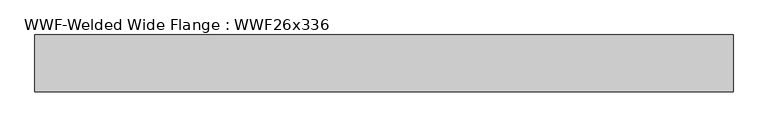
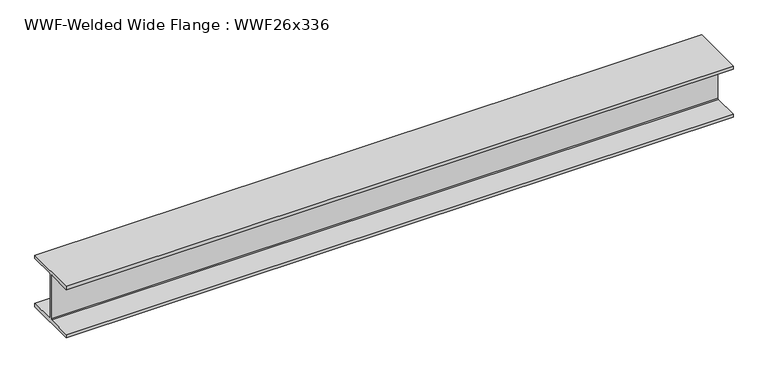
"""IFC4 building model written with IfcOpenShell, lengths in millimetres: beam geometry, WWF-Welded Wide Flange : WWF26x336."""

import ifcopenshell
import ifcopenshell.guid

model = None  # the IFC model being written
_history = None  # IfcOwnerHistory: only IFC2X3 demands one
_inside = {}  # id of a spatial element -> (the spatial element, [elements in it])
_under = {}  # id of a project, library or spatial element -> (it, [spatial elements below it])
_declared = {}  # id of a project -> (the project, [libraries it declares])
_typed = {}  # id of a type object -> (the type object, [elements of that type])
_made_of = {}  # id of a material, layer set ... -> (it, [elements and type objects made of it])


def new_model(schema):
    """Start an empty IFC model of exactly this schema.

    Asked for "IFC4X3", IfcOpenShell would pick the latest addendum, in which some entities
    have other attributes; the version numbers below select the first issue.
    IFC2X3 requires an IfcOwnerHistory on every rooted entity: one is made here for all.
    """
    global model, _history
    if schema == "IFC4X3":
        model = ifcopenshell.file(schema_version=(4, 3, 0, 0))
    else:
        model = ifcopenshell.file(schema=schema)
    _inside.clear()
    _under.clear()
    _declared.clear()
    _typed.clear()
    _made_of.clear()
    _history = None
    if model.schema == "IFC2X3":
        org = make("IfcOrganization", Name="unknown")
        user = make(
            "IfcPersonAndOrganization",
            ThePerson=make("IfcPerson", FamilyName="unknown"),
            TheOrganization=org,
        )
        app = make(
            "IfcApplication",
            ApplicationDeveloper=org,
            Version="unknown",
            ApplicationFullName="unknown",
            ApplicationIdentifier="unknown",
        )
        _history = make(
            "IfcOwnerHistory",
            OwningUser=user,
            OwningApplication=app,
            ChangeAction="ADDED",
            CreationDate=0,
        )
    return model


def make(cls, **values):
    """One entity of the class cls with the attributes given. An attribute that is None is left unset."""
    return model.create_entity(
        cls, **{name: value for name, value in values.items() if value is not None}
    )


def rooted(cls, **values):
    """An entity with a GlobalId (a new one), such as an element, a storey or a relation."""
    return make(cls, GlobalId=ifcopenshell.guid.new(), OwnerHistory=_history, **values)


def si_unit(unit_type, name, prefix=None):
    """IfcSIUnit, for example si_unit("LENGTHUNIT", "METRE", prefix="MILLI")."""
    return make("IfcSIUnit", UnitType=unit_type, Prefix=prefix, Name=name)


def assignment(units):
    """IfcUnitAssignment: the units of a project."""
    return None if units is None else make("IfcUnitAssignment", Units=units)


def point(xyz):
    """IfcCartesianPoint."""
    return None if xyz is None else make("IfcCartesianPoint", Coordinates=xyz)


def direction(xyz):
    """IfcDirection."""
    return None if xyz is None else make("IfcDirection", DirectionRatios=xyz)


def frame(location, z_axis=None, x_axis=None):
    """IfcAxis2Placement3D, a coordinate frame: its origin and axes. An axis left out is left unset."""
    return make(
        "IfcAxis2Placement3D",
        Location=point(location),
        Axis=direction(z_axis),
        RefDirection=direction(x_axis),
    )


def origin():
    """The frame at (0, 0, 0) with its axes left unset."""
    return frame((0.0, 0.0, 0.0))


def place(relative_to, where):
    """IfcLocalPlacement: puts the frame where relative to a parent placement (None: the world)."""
    return make(
        "IfcLocalPlacement", PlacementRelTo=relative_to, RelativePlacement=where
    )


def context(
    kind, dimensions, precision=None, world=None, true_north=None, identifier=None
):
    """IfcGeometricRepresentationContext, for example the 3D "Model" context."""
    return make(
        "IfcGeometricRepresentationContext",
        ContextIdentifier=identifier,
        ContextType=kind,
        CoordinateSpaceDimension=dimensions,
        Precision=precision,
        WorldCoordinateSystem=world,
        TrueNorth=true_north,
    )


def project(units=None, contexts=None):
    """IfcProject with its units and contexts."""
    return rooted(
        "IfcProject",
        Name="project",
        RepresentationContexts=contexts,
        UnitsInContext=assignment(units),
    )


def spatial(cls, under=None, at=None, **own):
    """A site, building, storey or space (cls), placed at a placement, below another one or the project."""
    s = rooted(cls, ObjectPlacement=at, **own)
    if under is not None:
        _under.setdefault(under.id(), (under, []))[1].append(s)
    return s


def polyline(points):
    """IfcPolyline through the points."""
    return make("IfcPolyline", Points=[point(p) for p in points])


def outline(outer, holes=None, kind="AREA"):
    """IfcArbitraryClosedProfileDef: a profile drawn as a closed curve; with holes, ...WithVoids."""
    if holes is None:
        return make("IfcArbitraryClosedProfileDef", ProfileType=kind, OuterCurve=outer)
    return make(
        "IfcArbitraryProfileDefWithVoids",
        ProfileType=kind,
        OuterCurve=outer,
        InnerCurves=holes,
    )


def extrude(swept, where, along, depth):
    """IfcExtrudedAreaSolid: the profile swept, set in the frame where, extruded along a direction by depth."""
    return make(
        "IfcExtrudedAreaSolid",
        SweptArea=swept,
        Position=where,
        ExtrudedDirection=direction(along),
        Depth=depth,
    )


def shape(context_of_items, identifier, shape_type, items):
    """IfcShapeRepresentation: the items that make up one representation, for example the "Body"."""
    return make(
        "IfcShapeRepresentation",
        ContextOfItems=context_of_items,
        RepresentationIdentifier=identifier,
        RepresentationType=shape_type,
        Items=items,
    )


def source(mapping_origin, context_of_items, identifier, shape_type, items):
    """IfcRepresentationMap: a shape defined once, which mapped items show again and again."""
    return make(
        "IfcRepresentationMap",
        MappingOrigin=mapping_origin,
        MappedRepresentation=shape(context_of_items, identifier, shape_type, items),
    )


def transform(
    local_origin,
    x_axis=None,
    y_axis=None,
    z_axis=None,
    scale=None,
    scale2=None,
    scale3=None,
    uniform=True,
):
    """IfcCartesianTransformationOperator3D, or its non-uniform kind. x_axis, y_axis, z_axis: its Axis1, 2, 3."""
    if uniform:
        return make(
            "IfcCartesianTransformationOperator3D",
            Axis1=direction(x_axis),
            Axis2=direction(y_axis),
            LocalOrigin=point(local_origin),
            Scale=scale,
            Axis3=direction(z_axis),
        )
    return make(
        "IfcCartesianTransformationOperator3DnonUniform",
        Axis1=direction(x_axis),
        Axis2=direction(y_axis),
        LocalOrigin=point(local_origin),
        Scale=scale,
        Axis3=direction(z_axis),
        Scale2=scale2,
        Scale3=scale3,
    )


def mapped(mapping_source, mapping_target):
    """IfcMappedItem: shows the shape of a source again, moved by a transform."""
    return make(
        "IfcMappedItem", MappingSource=mapping_source, MappingTarget=mapping_target
    )


def made_of(thing, what):
    """Note that an element or type object is made of a material, layer set ...; save() writes the relation."""
    if what is not None:
        _made_of.setdefault(what.id(), (what, []))[1].append(thing)
    return thing


def element(
    cls,
    number,
    at=None,
    inside=None,
    cuts=None,
    type_object=None,
    material=None,
    context=None,
    identifier="Body",
    shape_type=None,
    held_by="IfcProductDefinitionShape",
    body=None,
    shapes=None,
    **own,
):
    """One element of the class cls, such as IfcWall. Its Tag is "e" and its number.

    at: its placement. inside: the storey or other place that contains it. cuts: it is an
    opening in that element (IfcRelVoidsElement). A single representation is given by context,
    identifier, shape_type and body (its items); several are given by shapes. held_by: the class
    of the entity that holds the representations. save() writes the other relations.
    """
    e = rooted(cls, Tag="e%d" % number, ObjectPlacement=at, **own)
    if body is not None:
        shapes = [shape(context, identifier, shape_type, body)]
    if shapes is not None:
        e.Representation = make(held_by, Representations=shapes)
    if inside is not None:
        _inside.setdefault(inside.id(), (inside, []))[1].append(e)
    if cuts is not None:
        rooted(
            "IfcRelVoidsElement", RelatingBuildingElement=cuts, RelatedOpeningElement=e
        )
    if type_object is not None:
        _typed.setdefault(type_object.id(), (type_object, []))[1].append(e)
    return made_of(e, material)


def aggregate(whole, parts):
    """IfcRelAggregates: a whole, such as a stair, and the parts it consists of."""
    return rooted("IfcRelAggregates", RelatingObject=whole, RelatedObjects=parts)


def save(model, path):
    """Write the relations noted so far, then the file.

    IfcRelAggregates (storeys below a building ...), IfcRelContainedInSpatialStructure (elements
    in a storey), IfcRelDefinesByType, IfcRelAssociatesMaterial and IfcRelDeclares: one each for
    every whole, place, type object, material and project.
    """
    for whole, parts in _under.values():
        aggregate(whole, parts)
    for where, things in _inside.values():
        rooted(
            "IfcRelContainedInSpatialStructure",
            RelatedElements=things,
            RelatingStructure=where,
        )
    for kind, things in _typed.values():
        rooted("IfcRelDefinesByType", RelatedObjects=things, RelatingType=kind)
    for what, things in _made_of.values():
        rooted("IfcRelAssociatesMaterial", RelatedObjects=things, RelatingMaterial=what)
    for by, libraries in _declared.values():
        rooted("IfcRelDeclares", RelatingContext=by, RelatedDefinitions=libraries)
    model.write(path)


def wwf_welded_wide_flange_wwf26x336_8fc15e60(model_context):
    return source(origin(), model_context, "Body", "SweptSolid", [
        extrude(outline(polyline([(324.993, -284.988), (324.993, -324.993), (-324.993, -324.993), (-324.993, -284.988), (-20.6375, -284.988), (-9.9949, -274.3454), (-9.9949, 274.3454), (-20.6375, 284.988), (-324.993, 284.988), (-324.993, 324.993), (324.993, 324.993), (324.993, 284.988), (20.6375, 284.988), (9.9949, 274.3454), (9.9949, -274.3454), (20.6375, -284.988), (324.993, -284.988)])), frame((-3827.7582557, 0.0, 0.0), z_axis=(1.0, 0.0, 0.0), x_axis=(0.0, 1.0, 0.0)), (0.0, 0.0, 1.0), 7985.2376991),
    ])


if __name__ == "__main__":
    model = new_model("IFC4")
    model_context = context("Model", 3, world=origin())
    ifc_project = project(units=[si_unit("LENGTHUNIT", "METRE", prefix="MILLI")], contexts=[model_context])
    site = spatial("IfcSite", under=ifc_project)
    building = spatial("IfcBuilding", under=site)
    placement = place(None, origin())
    wwf_welded_wide_flange_wwf26x336_shape = wwf_welded_wide_flange_wwf26x336_8fc15e60(model_context)
    element("IfcBeam", 1, ObjectType="WWF-Welded Wide Flange : WWF26x336", at=placement, inside=building, context=model_context, shape_type="MappedRepresentation", body=[
        mapped(wwf_welded_wide_flange_wwf26x336_shape, transform((0.0, 0.0, 0.0), x_axis=(1.0, 0.0, 0.0), y_axis=(0.0, 1.0, 0.0), z_axis=(0.0, 0.0, 1.0))),
    ])
    save(model, "model.ifc")

# Revit data of these elements
# Type "WWF-Welded Wide Flange : WWF26x336"
#   Assembly Code = "B10"
#   Nominal d = "12"
#   W = 336
#   Length [instance default] = 1524 mm
#   bf = 649.986 mm
#   d = 649.986 mm
#   k = 20.638 mm
#   tf = 40.005 mm
#   tw = 19.99 mm
#   A = 0.0635483 m²
#   Structural Material [instance default] = Steel ASTM A572
# Element 1 (IfcBeam, "WWF-Welded Wide Flange : WWF26x336")
#   Structural Material = Metal - Steel 43-275
#   Materials on its faces: "Metal - Steel 43-275"
# Materials
#   "Steel ASTM A572": class "Metal", colour RGB 247 247 247, transparency 0, Description = "Structural steel, high strength low alloy, ASTM - A572 - 50", Cost = 0
#   "Metal - Steel 43-275": class "Metal", colour RGB 247 247 247, transparency 0, Cost = 0
